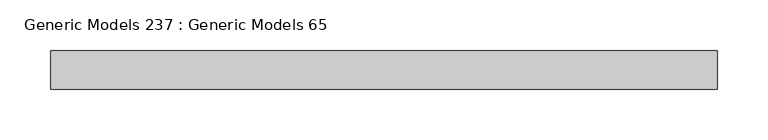
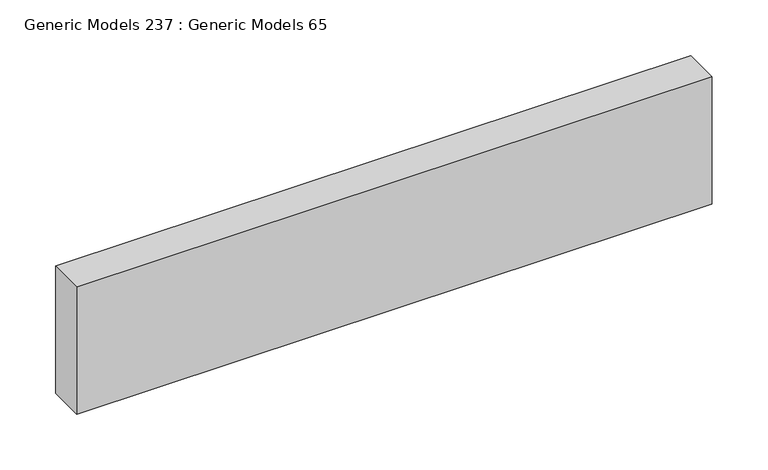
"""IFC4 building model written with IfcOpenShell, lengths in millimetres: proxy geometry, Generic Models 237 : Generic Models 65."""

from ifc_helpers import new_model, si_unit, frame, origin, place, context, project, spatial, polyline, outline, extrude, source, transform, mapped, element, save


def generic_models_237_generic_models_65_1df05f16(model_context):
    return source(origin(), model_context, "Body", "SweptSolid", [
        extrude(outline(polyline([(48469.55, 592.1375), (48469.55, 630.2375), (49128.3625, 630.2375), (49128.3625, 592.1375), (48469.55, 592.1375)])), frame((0.0, 0.0, 5507.83125), z_axis=(0.0, 0.0, 1.0), x_axis=(1.0, 0.0, 0.0)), (0.0, 0.0, 1.0), 139.7),
    ])


if __name__ == "__main__":
    model = new_model("IFC4")
    model_context = context("Model", 3, world=origin())
    ifc_project = project(units=[si_unit("LENGTHUNIT", "METRE", prefix="MILLI")], contexts=[model_context])
    site = spatial("IfcSite", under=ifc_project)
    building = spatial("IfcBuilding", under=site)
    placement = place(None, origin())
    generic_models_237_generic_models_65_shape = generic_models_237_generic_models_65_1df05f16(model_context)
    element("IfcBuildingElementProxy", 1, Name="Generic Models 237 : Generic Models 65", ObjectType="Generic Models 237 : Generic Models 65", at=placement, inside=building, context=model_context, shape_type="MappedRepresentation", body=[
        mapped(generic_models_237_generic_models_65_shape, transform((0.0, 0.0, 0.0), x_axis=(1.0, 0.0, 0.0), y_axis=(0.0, 1.0, 0.0), z_axis=(0.0, 0.0, 1.0))),
    ])
    save(model, "model.ifc")

# Revit data of these elements
# Element 1 (IfcBuildingElementProxy, "Generic Models 237 : Generic Models 65")
#   Materials on its faces: "WOOD JOIST AS SPECIFIED"
# Materials
#   "WOOD JOIST AS SPECIFIED": class "Wood", colour RGB 234 198 147, transparency 0, Description = "Pinus Echinata", Cost = 0
